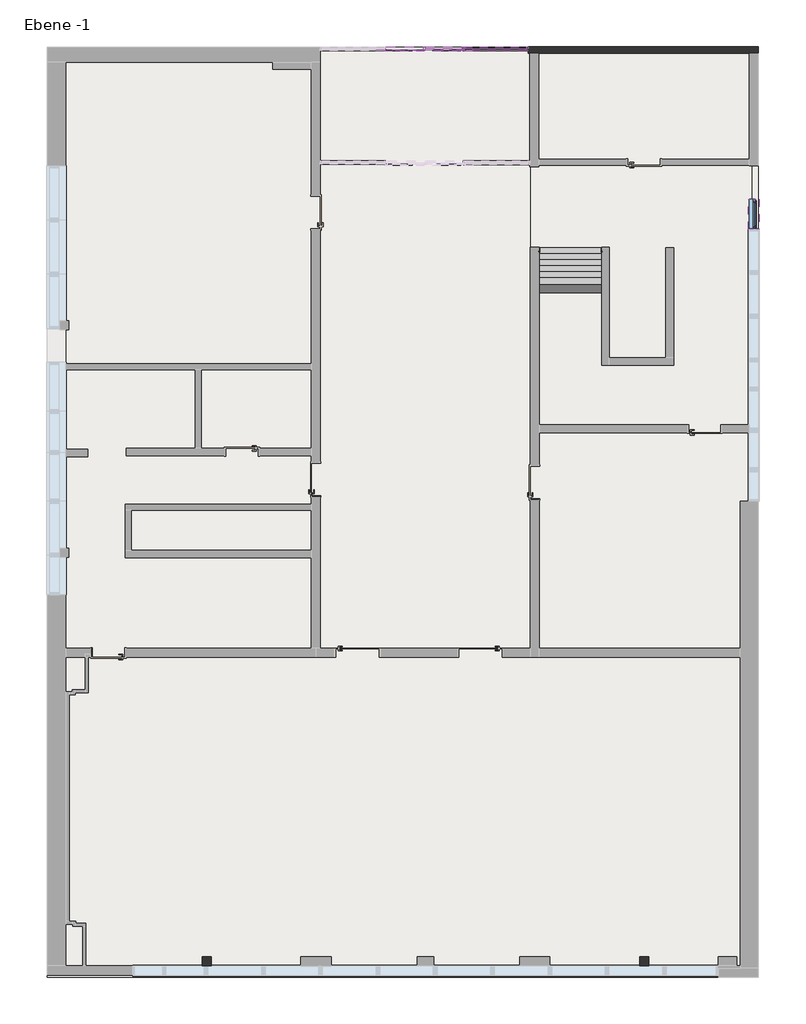
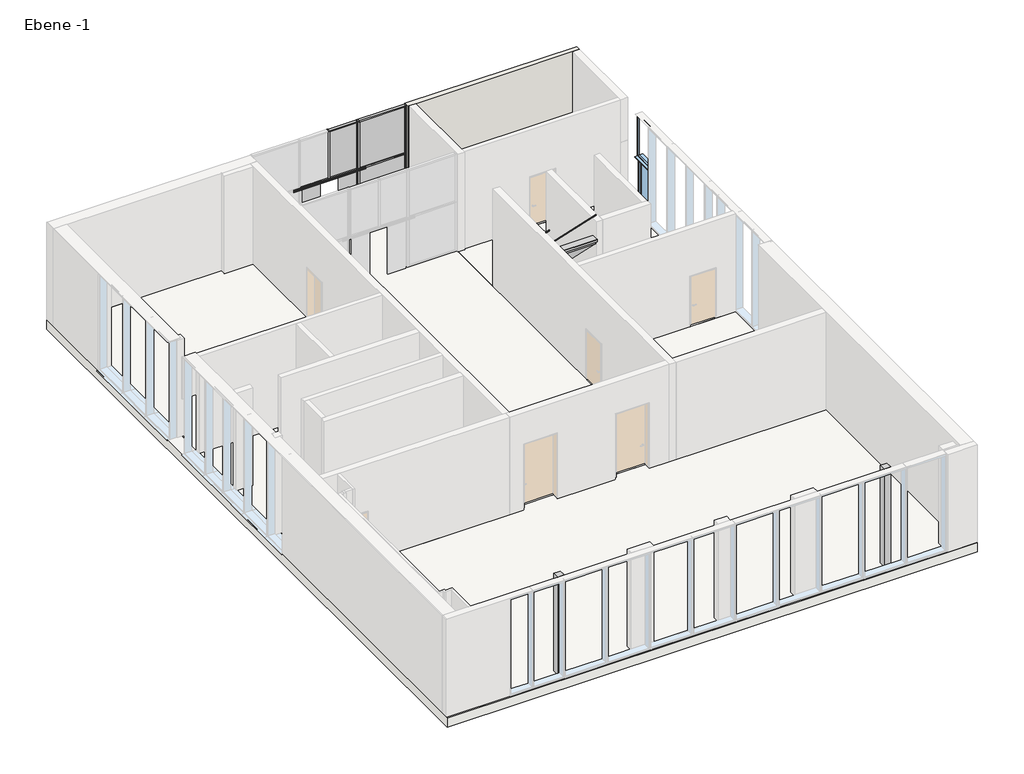
# One storey, part 3 of 3: 14 members, 8 slabs, 5 plates, 2 columns, 2 railings, 2 windows, 1 stair flight, 1 wall.
# Revit data of these elements (continued)
# Project information (continued)
#   Projektstatus = "Projektstatus"
#   Kundenname = "Bauherr"
#   Projektadresse = "Projektadresse"
#   Projektname = "Projektname"
#   Projektnummer = "Projektnummer"
#   Verfasser Firma 1 = "Firma 1"
#   Verfasser Firma 2 = "Firma 2"
#   Verfasser PLZ Ort = "PLZ Ort"
#   Verfasser Strasse = "Strasse"
#   Verfasser Telefon = "Telefon"
#   Verfasser Telefax = "Telefax"
#   Verfasser eMail = "E-Mail"
# Type "STB Stütze - rechteckig : STB 30 x 30"
#   Breite = 0.300 m
#   Tiefe = 0.300 m
#   Structural Material [instance default] = Stahlbeton - Ortbeton
# Type "Pfosten rechteckig : 6 x 12"
#   built-in parameter 1007304 = 0.393701 (stored number, unit not read)
#   built-in parameter 1007301 = 0.0984252 (stored number, unit not read)
#   built-in parameter 1007300 = 0.0984252 (stored number, unit not read)
# Type "Türelement 2-flg - Schiebeflügel : Standard"
#   Construction Type Id = "GSP4R"
#   Analytic Construction = "1/8 Zoll Pilkington-Verglasung einfach"
#   Visual Light Transmittance = 0.9
#   Thermal Resistance (R) = 0.270117 (m²·K)/W
#   Solar Heat Gain Coefficient = 0.86
#   Öffnungswert [instance default] = 0.400 m
#   Heat Transfer Coefficient (U) = 6.7069 W/(m²·K)
#   Länge Schiene [instance default] = 3.200 m
#   Halbe Breite [instance default] = 0.800 m
#   Versatz zur Achse [instance default] = 0.100 m
#   Gesamtbreite Tür [instance default] = 1.600 m
#   Schiene anzeigen [instance default] = yes
#   Prozent [instance default] = 50
#   Geöffnet in % [instance default] = 50
#   Schiene [instance default] = none
#   Tür [instance default] = none
# Type "Systemelement : Verglasung"
#   Construction Type Id = "GSP4R"
#   Analytic Construction = "1/8 Zoll Pilkington-Verglasung einfach"
#   Visual Light Transmittance = 0.9
#   Solar Heat Gain Coefficient = 0.86
#   Heat Transfer Coefficient (U) = 6.7069 W/(m²·K)
# Type "Holzhandlauf"
#   Assembly Code = ""
#   built-in parameter 1008612 = 0.0416667 (stored number, unit not read)
#   built-in parameter 1008611 = 0.0416667 (stored number, unit not read)
#   built-in parameter 1008609 = 0.333333 (stored number, unit not read)
#   built-in parameter 1008604 = 0.166667 (stored number, unit not read)
#   built-in parameter 1008603 = 0.166667 (stored number, unit not read)
#   Railing Height = 0.900 m
#   built-in parameter 1008630 = 2
#   built-in parameter 1008610 = 2
# Type "Fließen"
#   Function = 0
#   Layers, outside or top first: 0.020 m "Decke - Fliesen 25 x 25" (function 1)
# Type "PVC"
#   Function = 0
#   Layers, outside or top first: 0.020 m "Standard - Fußboden" (function 1)
# Type "Parkett"
#   Function = 0
#   Layers, outside or top first: 0.020 m "Holz - Parkett" (function 1)
# Type "STB 30"
#   Function = 0
#   Layers, outside or top first: 0.300 m "Stahlbeton - Ortbeton" (function 1); 0.060 m "Wärmedämmung - hart" (function 3); 0.060 m "Wärmedämmung - weich" (function 3)
# Type "STB 21.0 - Sichtbeton 1"
#   Type Comments = "Stahlbeton Sichtbeton"
#   Description = "Stahlbeton (Sichtbeton) 30.0"
#   Layers, outside or top first: 0.215 m "Stahlbeton - Sichtbeton (1)" (function 1)
# Type "Fenster - Festverglasung : Feste Verglasung 1.0 x2 2"
#   Type Mark = "74"
#   Operation = "SinglePanel"
#   Keynote = "16.05.01"
#   Visual Light Transmittance = 0.9
#   Solar Heat Gain Coefficient = 0.78
#   Rough Width = 1.000 m
#   Rough Height = 2.000 m
#   Heat Transfer Coefficient (U) = 3.6886 W/(m²·K)
#   Rahmentiefe = 0.050 m
#   Rahmenhöhe unten = 0.080 m
#   Höhe oberer  Rahmen = 0.080 m
#   Rahmenbreite = 0.060 m
#   Height = 2.000 m
#   Einbautiefe (von außen) [instance default] = 0.080 m
#   Width = 1.000 m
#   Wall Closure = 2
#   Bild [instance default] = none
#   Glas [instance default] = none
#   Innere Fensterbank [instance default] = none
#   Äußere Fensterbank [instance default] = none
#   Construction Type Id = ""
#   Analytic Construction = (empty or 0)
# Type "Fenstertür 1-flg : 1.80 x  1"
#   Type Mark = "73"
#   Operation = "SinglePanel"
#   Construction Type Id = "GSP4R"
#   Keynote = "16.05.01"
#   Analytic Construction = "1/8 Zoll Pilkington-Verglasung einfach"
#   Visual Light Transmittance = 0.9
#   Thermal Resistance (R) = 0.1491 (m²·K)/W
#   Solar Heat Gain Coefficient = 0.86
#   Rough Width = 1.000 m
#   Rough Height = 2.600 m
#   Heat Transfer Coefficient (U) = 6.7069 W/(m²·K)
#   Rahmentiefe = 0.080 m
#   Rahmenhöhe - unten = 0.080 m
#   Rahmenhöhe - oben = 0.080 m
#   Rahmenbreite = 0.080 m
#   Height = 2.600 m
#   Tiefe Flügel = 0.060 m
#   Flügelbreite = 0.060 m
#   Einbautiefe (von außen) [instance default] = 0.080 m
#   Width = 1.000 m
#   Kippflügel [instance default] = yes
#   Drehflügel im Grundriss darstellen [instance default] = yes
#   Drehflügel 1 [instance default] = yes
#   Rahmen 1 [instance default] = none
#   Glas [instance default] = none
#   Flügel [instance default] = none
#   Fensterbank Außenseite [instance default] = none
#   Wall Closure = (empty or 0)
# Elements 1, 2 (IfcColumn, "STB Stütze - rechteckig : STB 30 x 30")
#   Comments = ""
#   Structural Material = Stahlbeton - Ortbeton
#   Phase Created = Phase 1
#   Materials on its faces: "Stahlbeton - Ortbeton"
# Elements 3, 4, 5, 6, 7, 8, 9, 10, 11, 12, 13, 14, 15, 16 (IfcMember, "Pfosten rechteckig : 6 x 12")
#   Phase Created = Phase 1
#   Materials on its faces: "Metall - verzinkt"
# Elements 17, 18 (IfcPlate, "Türelement 2-flg - Schiebeflügel : Standard")
#   Öffnungswert = 0.400 m
#   Versatz zur Achse = 0.100 m
#   Länge Schiene = 3.200 m
#   Halbe Breite = 0.800 m
#   Gesamtbreite Tür = 1.600 m
#   Schiene anzeigen = yes
#   Prozent = 50
#   Geöffnet in % = 50
#   Tür = none
#   Schiene = none
#   Phase Created = Phase 1
#   Materials on its faces: "Glas"
# Elements 19, 20, 21 (IfcPlate, "Systemelement : Verglasung")
#   Phase Created = Phase 1
#   Materials on its faces: "Glas"
# Elements 22, 23 (IfcRailing, "Holzhandlauf")
#   Phase Created = Phase 1
#   Materials on its faces: "Holz - Birke"
# Element 24 (IfcSlab, "Fließen")
#   built-in parameter 1001955 = -1.5708 (stored number, unit not read)
#   Height Offset From Level = 0.000 m
#   Phase Created = Phase 1
#   Materials on its faces: "Decke - Fliesen 25 x 25"
# Element 25 (IfcSlab, "PVC")
#   built-in parameter 1001955 = -1.5708 (stored number, unit not read)
#   Height Offset From Level = 0.000 m
#   Phase Created = Phase 1
#   Materials on its faces: "Standard - Fußboden"
# Elements 26, 27, 28, 29 (IfcSlab, "PVC")
#   Height Offset From Level = 0.000 m
#   Phase Created = Phase 1
#   Materials on its faces: "Standard - Fußboden"
# Element 30 (IfcSlab, "Parkett")
#   built-in parameter 1001955 = -1.5708 (stored number, unit not read)
#   Height Offset From Level = 0.000 m
#   Phase Created = Phase 1
#   Materials on its faces: "Holz - Parkett"
# Element 31 (IfcSlab, "STB 30")
#   Height Offset From Level = -0.020 m
#   built-in parameter 1001954 = 1
#   Phase Created = Phase 1
#   Materials on its faces: "Wärmedämmung - weich", "Stahlbeton - Ortbeton"
# Element 32 (IfcStairFlight, "Holzauftritt 30 mm, Trittüberstand 30 mm")
#   Phase Created = Phase 1
#   Materials on its faces: "Holz - Birke", "Stahlbeton - Fertigbeton"
# Element 33 (IfcWall, "STB 21.0 - Sichtbeton 1")
#   Comments = ""
#   Top Offset = 0.000 m
#   Base Offset = 0.000 m
#   wall height = 4.58484 m
#   Phase Created = Phase 1
#   Base Constraint = Ebene -1
#   Top Constraint = Ebene 1
#   Materials on its faces: "Stahlbeton - Sichtbeton (1)", "Stahlbeton - Sichtbeton (2)"
# Element 34 (IfcWindow, "Fenster - Festverglasung : Feste Verglasung 1.0 x2 2")
#   Mark = "51"
#   Einbautiefe (von außen) = 0.080 m
#   Äußere Fensterbank = none
#   Innere Fensterbank = none
#   Glas = none
#   Bild = none
#   Phase Created = Phase 1
#   Materials on its faces: "Kunststoff - Weiß", "Holz - Birke"
# Element 35 (IfcWindow, "Fenstertür 1-flg : 1.80 x  1")
#   Mark = "50"
#   Einbautiefe (von außen) = 0.128689 m
#   Kippflügel = yes
#   Drehflügel im Grundriss darstellen = yes
#   Drehflügel 1 = yes
#   Rahmen 1 = none
#   Glas = none
#   Flügel = none
#   Fensterbank Außenseite = none
#   Phase Created = Phase 1
#   Materials on its faces: "Kunststoff - Weiß", "Glas"
# Materials
#   "Stahlbeton - Ortbeton": class "Beton", colour RGB 247 247 247, transparency 0, Cost = 0
#   "Decke - Fliesen 25 x 25": class "Keramik", colour RGB 247 247 247, transparency 0, Cost = 0
#   "Standard - Fußboden": class "Farbe 1", colour RGB 172 172 172, transparency 0, Cost = 0
#   "Holz - Parkett": class "Holz", colour RGB 223 173 112, transparency 0, Cost = 0
#   "Wärmedämmung - hart": class "Stuck", colour RGB 255 255 255, transparency 0, Description = "Äußere Oberfläche", Cost = 0
#   "Wärmedämmung - weich": class "Stuck", colour RGB 247 247 247, transparency 0, Description = "Äußere Oberfläche", Cost = 0
#   "Stahlbeton - Sichtbeton (1)": class "Beton", colour RGB 192 192 192, transparency 0, Cost = 0
#   "Metall - verzinkt": class "Allgemeines", colour RGB 200 200 200, transparency 0, Cost = 0
#   "Glas": class "Glas", colour RGB 0 0 255, transparency 0.75, Comments = "Render-Darstellung nicht aktualisiert ", Cost = 0
#   "Holz - Birke": class "Holz", colour RGB 213 164 103, transparency 0, Cost = 0
#   "Stahlbeton - Fertigbeton": class "Beton", colour RGB 247 247 247, transparency 0, Cost = 0
#   "Stahlbeton - Sichtbeton (2)": class "Beton", colour RGB 192 192 192, transparency 0, Cost = 0
#   "Kunststoff - Weiß": class "Kunststoff", colour RGB 249 249 249, transparency 0, Cost = 0
